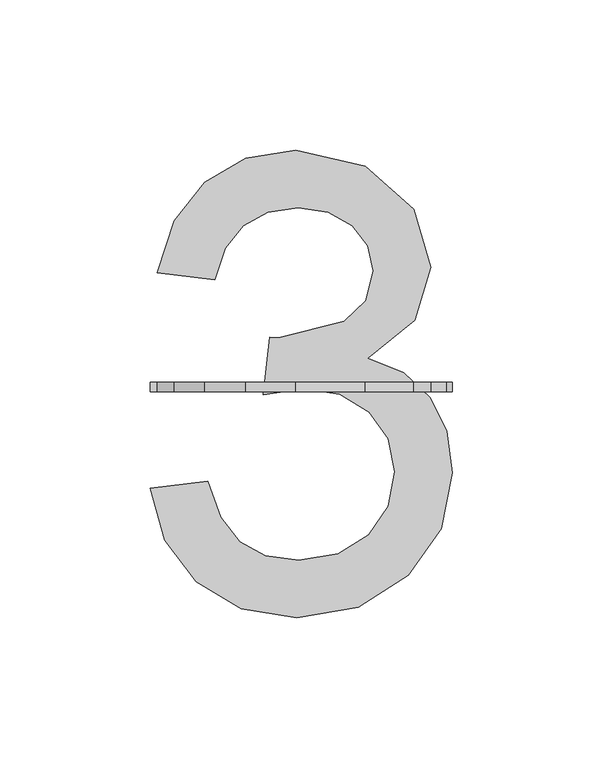
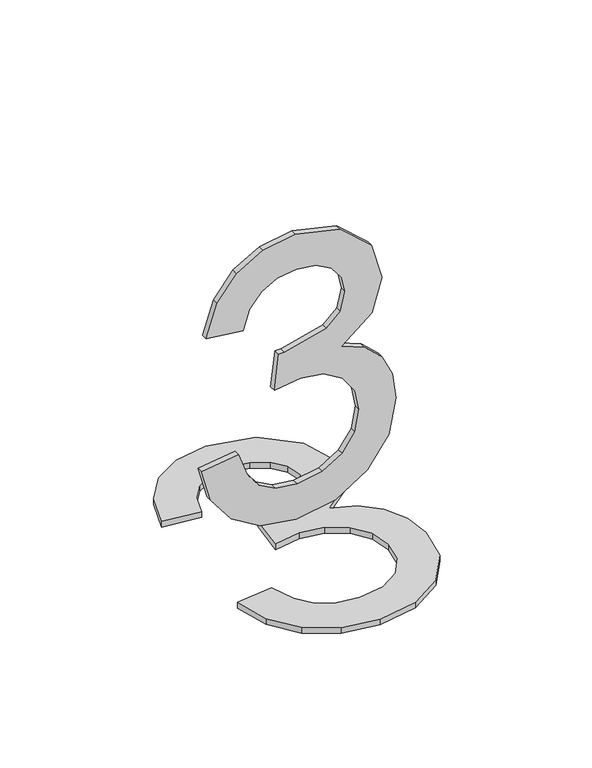
"""IFC4 building model written with IfcOpenShell, lengths in millimetres: proxy geometry, Grid Number1_FedEx : Grid Number1_FedEx."""

from ifc_helpers import new_model, si_unit, frame, origin, origin_with_axes, place, context, project, spatial, polyline, outline, extrude, source, transform, mapped, element, save


def entourage_107cf9cf(model_context):
    return source(origin(), model_context, "Body", "SweptSolid", [
        extrude(outline(polyline([(-157.1123024, 187.250035), (-137.9753753, 189.6421509), (-133.6910584, 177.616162), (-127.4164263, 169.4960499), (-118.8431203, 164.8706696), (-107.6627818, 163.3288761), (-94.5435213, 165.4500101), (-84.4144056, 171.8134122), (-77.9388731, 181.3071221), (-75.7803623, 192.8191798), (-77.9201847, 203.7472248), (-84.3396519, 212.610201), (-94.0576227, 218.4830324), (-106.0929558, 220.4406429), (-119.5112308, 218.3475415), (-117.3807526, 237.4844686), (-114.3158541, 237.2602077), (-92.5999271, 242.7545989), (-85.3675142, 249.7253741), (-82.9567099, 259.6489173), (-84.7040758, 267.9138646), (-89.9461735, 274.61833), (-97.944811, 279.0614984), (-107.9617963, 280.5425545), (-117.99747, 279.0474821), (-126.2016799, 274.5622648), (-132.1913138, 267.0869027), (-135.5832594, 256.6213957), (-154.7201865, 259.0135115), (-149.0856323, 276.1975003), (-139.0593028, 289.0270905), (-125.3420133, 297.0163838), (-108.6345789, 299.6794816), (-85.5543983, 294.4280397), (-69.4076161, 280.0753444), (-63.8197829, 260.7702216), (-69.12729, 243.128367), (-84.8255505, 230.4576282), (-72.8462826, 225.6173312), (-63.9692901, 217.3757444), (-58.4748989, 206.1813896), (-56.6434352, 192.4827885), (-60.3063627, 173.8317599), (-71.295145, 158.2456299), (-87.8811048, 147.7053692), (-108.3355644, 144.191949), (-126.8370857, 147.1914381), (-141.8999404, 156.1899053), (-152.3747916, 169.9539158), (-157.1123024, 187.250035)])), origin_with_axes(), (0.0, 0.0, 1.0), 3.175),
        extrude(outline(polyline([(55.1458633, -157.1123024), (37.8497441, -152.3747916), (24.0857336, -141.8999404), (15.0872664, -126.8370857), (12.0877774, -108.3355644), (15.6011976, -87.8811048), (26.1414582, -71.295145), (41.7275883, -60.3063627), (60.3786168, -56.6434352), (74.0772179, -58.4748989), (85.2715727, -63.9692901), (93.5131595, -72.8462826), (98.3534565, -84.8255505), (111.0241953, -69.12729), (128.66605, -63.8197829), (147.9711727, -69.4076161), (162.323868, -85.5543983), (167.5753099, -108.6345789), (164.9122121, -125.3420133), (156.9229189, -139.0593028), (144.0933286, -149.0856323), (126.9093399, -154.7201865), (124.517224, -135.5832594), (134.982731, -132.1913138), (142.4580931, -126.2016799), (146.9433104, -117.99747), (148.4383828, -107.9617963), (146.9573267, -97.944811), (142.5141583, -89.9461735), (135.8096929, -84.7040758), (127.5447456, -82.9567099), (117.6212024, -85.3675142), (110.6504272, -92.5999271), (105.156036, -114.3158541), (105.3802969, -117.3807526), (86.2433698, -119.5112308), (88.3364712, -106.0929558), (86.3788607, -94.0576227), (80.5060294, -84.3396519), (71.6430531, -77.9201847), (60.7150081, -75.7803623), (49.2029504, -77.9388731), (39.7092405, -84.4144056), (33.3458385, -94.5435213), (31.2247044, -107.6627818), (32.7664979, -118.8431203), (37.3918782, -127.4164263), (45.5119903, -133.6910584), (57.5379792, -137.9753753), (55.1458633, -157.1123024)])), frame((0.0, 219.3456765, 0.0), z_axis=(0.0, 1.0, 0.0), x_axis=(0.0, 0.0, 1.0)), (0.0, 0.0, 1.0), 3.175),
    ])


if __name__ == "__main__":
    model = new_model("IFC4")
    model_context = context("Model", 3, world=origin())
    ifc_project = project(units=[si_unit("LENGTHUNIT", "METRE", prefix="MILLI")], contexts=[model_context])
    site = spatial("IfcSite", under=ifc_project)
    building = spatial("IfcBuilding", under=site)
    placement = place(None, origin())
    entourage_shape = entourage_107cf9cf(model_context)
    element("IfcBuildingElementProxy", 1, Name="Grid Number1_FedEx : Grid Number1_FedEx", ObjectType="Grid Number1_FedEx : Grid Number1_FedEx", at=placement, inside=building, context=model_context, shape_type="MappedRepresentation", body=[
        mapped(entourage_shape, transform((0.0, 0.0, 0.0), x_axis=(1.0, 0.0, 0.0), y_axis=(0.0, 1.0, 0.0), z_axis=(0.0, 0.0, 1.0))),
    ])
    save(model, "model.ifc")

# Revit data of these elements
# Type "Grid Number1_FedEx : Grid Number1_FedEx"
#   Grid [instance default] = "S.8"
#   Label Width [instance default] = 1' - 0"
#   Half Box Width2 [instance default] = 0' - 6.13846"
#   Half Box Width [instance default] = 0' - 6"
#   Robust [instance default] = yes
#   Height = 0
#   Assembly Code = ""
# Element 1 (IfcBuildingElementProxy, "Grid Number1_FedEx : Grid Number1_FedEx")
#   Grid = "3"
#   Robust = no
#   Materials on its faces: "Letter"
# Materials
#   "Letter": class "Unassigned", colour RGB 178 187 30, transparency 0, Comments = "Rendering appearance not upgraded "
